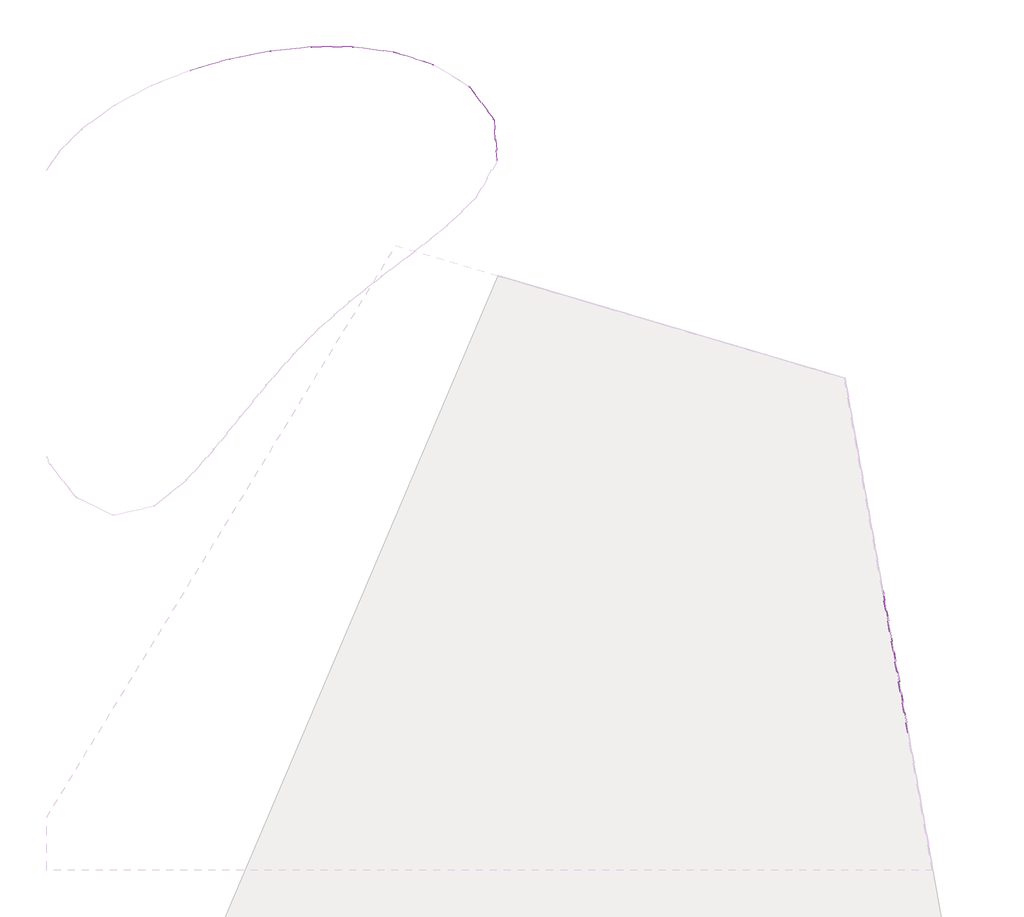
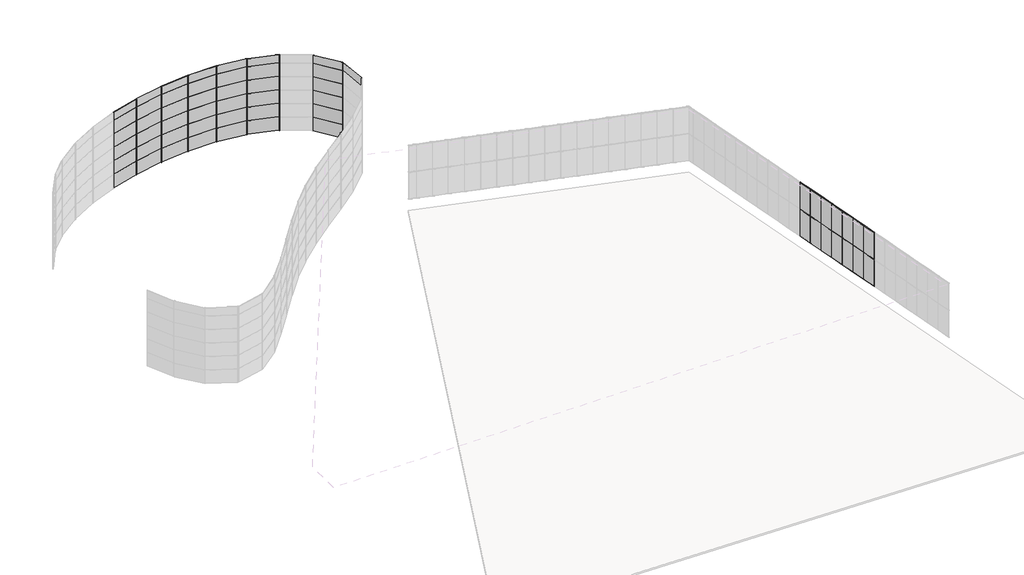
# One storey, part 7 of 8: 63 members, 57 plates.
# Revit data of these elements (continued)
# Type "Montante circular : 25 mm Raio"
#   built-in parameter 1007350 = 0.082021 (stored number, unit not read)
# Type "Painel do sistema : Envidraçado"
#   Construction Type Id = "GSP4R"
#   Analytic Construction = "Vidraça única Pilkington 1/8 pol"
#   Visual Light Transmittance = 0.9
#   Solar Heat Gain Coefficient = 0.86
#   Heat Transfer Coefficient (U) = 6.7069 W/(m²·K)
# Elements 1, 2, 3, 4, 5, 6, 7, 8, 9, 10, 11, 12, 13, 14, 15, 16, 17, 18, 19, 20, 21, 22, 23, 24, 25, 26, 27, 28, 29, 30, 31, 32, 33, 34, 35, 36, 37, 38, 39, 40, 41, 42, 43, 44, 45, 46, 47, 48, 49, 50, 51, 52, 53, 54, 55, 56, 57, 58, 59, 60, 61, 62, 63 (IfcMember, "Montante circular : 25 mm Raio")
#   Phase Created = Construção nova
#   Materials on its faces: "Alumín."
# Elements 64, 65, 66, 67, 68, 69, 70, 71, 72, 73, 74, 75, 76, 77, 78, 79, 80, 81, 82, 83, 84, 85, 86, 87, 88, 89, 90, 91, 92, 93, 94, 95, 96, 97, 98, 99, 100, 101, 102, 103, 104, 105, 106, 107, 108, 109, 110, 111, 112, 113, 114, 115, 116, 117, 118, 119, 120 (IfcPlate, "Painel do sistema : Envidraçado")
#   Phase Created = Construção nova
#   Materials on its faces: "Vidro"
# Materials
#   "Alumín.": class "Metal", colour RGB 247 247 247, transparency 0, Description = "Alumín. 6061", Cost = 0
#   "Vidro": class "Vidro", colour RGB 0 128 192, transparency 0.9, Description = "Vidro de sílica", Cost = 0
